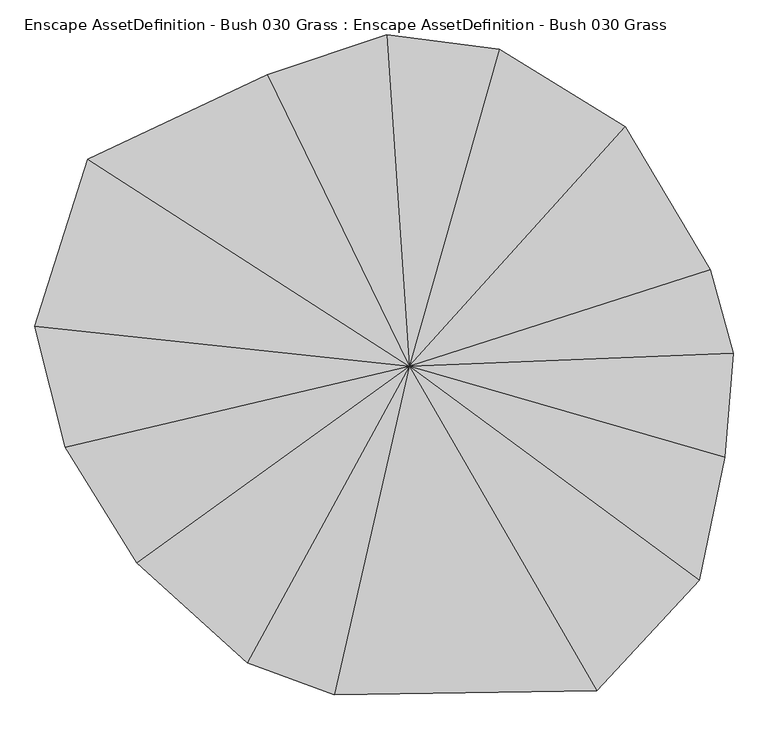
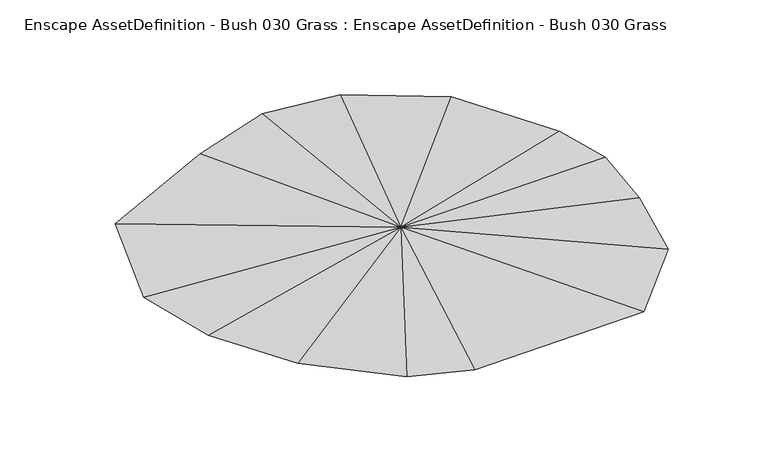
"""IFC4 building model written with IfcOpenShell, lengths in millimetres: geographic element geometry, Enscape AssetDefinition - Bush 030 Grass : Enscape AssetDefinition - Bush 030 Grass."""

from ifc_helpers import new_model, si_unit, origin, place, context, project, spatial, faceted_brep, source, transform, mapped, element, save


def enscape_assetdefinition_bush_030_grass_enscape_fc38328f(model_context):
    return source(origin(), model_context, "Body", "Brep", [
        faceted_brep([(46.6700345, 4.837607, 10.4857637), (-156.0632885, 421.6965139, 0.0005243), (-413.0132496, 301.0389209, 0.0), (14.2548708, 478.6814153, 0.0005243), (-488.4850383, 62.3530708, 0.0005243), (175.0823557, 458.5749507, 0.0), (355.5533588, 347.4667668, 0.0), (509.7507238, 23.7492062, 0.0005243), (-60.6722012, -464.8402035, 0.0), (-445.4378784, -110.6646508, 0.0), (-343.1681097, -275.8107185, 0.0), (-185.1303428, -419.0105796, 0.0005243), (315.0657415, -459.1831267, 0.0005243), (461.2535238, -301.1049926, 0.0), (498.0376065, -125.5266517, 0.0), (476.8353701, 142.9650038, 0.0)], [[[0, 1, 2]], [[0, 3, 1]], [[2, 1, 3]], [[0, 2, 4]], [[2, 3, 4]], [[0, 5, 3]], [[6, 3, 5]], [[7, 3, 6]], [[8, 3, 7]], [[4, 3, 8]], [[0, 4, 9]], [[4, 10, 9]], [[4, 8, 10]], [[0, 9, 10]], [[0, 10, 11]], [[10, 8, 11]], [[0, 11, 8]], [[0, 8, 12]], [[8, 13, 12]], [[8, 7, 13]], [[0, 12, 13]], [[0, 13, 14]], [[13, 7, 14]], [[0, 14, 7]], [[0, 7, 15]], [[0, 15, 6]], [[0, 6, 5]], [[7, 6, 15]]]),
    ])


if __name__ == "__main__":
    model = new_model("IFC4")
    model_context = context("Model", 3, world=origin())
    ifc_project = project(units=[si_unit("LENGTHUNIT", "METRE", prefix="MILLI")], contexts=[model_context])
    site = spatial("IfcSite", under=ifc_project)
    building = spatial("IfcBuilding", under=site)
    placement = place(None, origin())
    enscape_assetdefinition_bush_030_grass_enscape_shape = enscape_assetdefinition_bush_030_grass_enscape_fc38328f(model_context)
    element("IfcGeographicElement", 1, ObjectType="Enscape AssetDefinition - Bush 030 Grass : Enscape AssetDefinition - Bush 030 Grass", at=placement, inside=building, context=model_context, shape_type="MappedRepresentation", body=[
        mapped(enscape_assetdefinition_bush_030_grass_enscape_shape, transform((0.0, 0.0, 0.0), x_axis=(1.0, 0.0, 0.0), y_axis=(0.0, 1.0, 0.0), z_axis=(0.0, 0.0, 1.0))),
    ])
    save(model, "model.ifc")

# Revit data of these elements
# Type "Enscape AssetDefinition - Bush 030 Grass : Enscape AssetDefinition - Bush 030 Grass"
#   EnscapeAssetSource = "REMOTE"
#   EnscapeAssetId = "00026ee4-e1b1-4e5d-9a6f-71123b7d7688"
#   Height = 0.010486 m
#   EnscapeNativeAssetHeight = 0.010486 m
#   Default Elevation = 0
